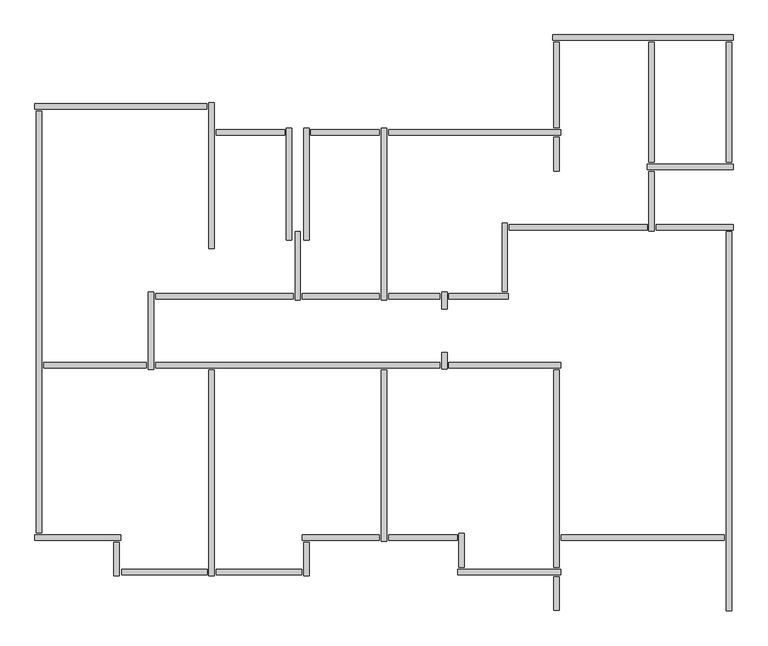
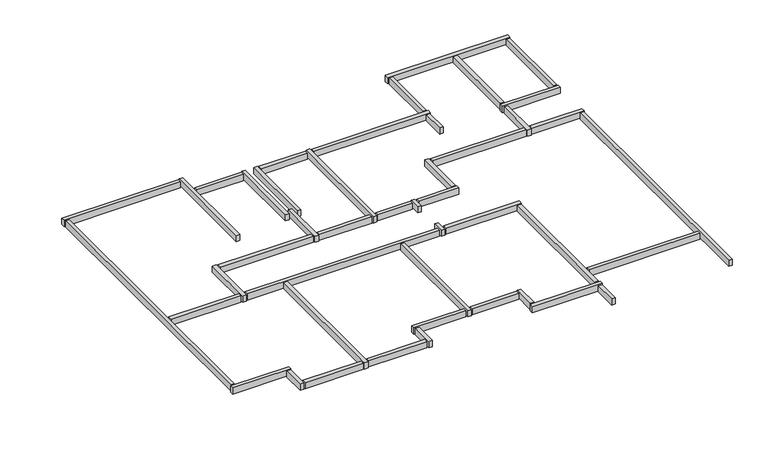
"""IFC4 building model written with IfcOpenShell, lengths in millimetres: beam geometry, Graute viga de respaldo18 : Graute viga de respaldo."""

import ifcopenshell
import ifcopenshell.guid

model = None  # the IFC model being written
_history = None  # IfcOwnerHistory: only IFC2X3 demands one
_inside = {}  # id of a spatial element -> (the spatial element, [elements in it])
_under = {}  # id of a project, library or spatial element -> (it, [spatial elements below it])
_declared = {}  # id of a project -> (the project, [libraries it declares])
_typed = {}  # id of a type object -> (the type object, [elements of that type])
_made_of = {}  # id of a material, layer set ... -> (it, [elements and type objects made of it])


def new_model(schema):
    """Start an empty IFC model of exactly this schema.

    Asked for "IFC4X3", IfcOpenShell would pick the latest addendum, in which some entities
    have other attributes; the version numbers below select the first issue.
    IFC2X3 requires an IfcOwnerHistory on every rooted entity: one is made here for all.
    """
    global model, _history
    if schema == "IFC4X3":
        model = ifcopenshell.file(schema_version=(4, 3, 0, 0))
    else:
        model = ifcopenshell.file(schema=schema)
    _inside.clear()
    _under.clear()
    _declared.clear()
    _typed.clear()
    _made_of.clear()
    _history = None
    if model.schema == "IFC2X3":
        org = make("IfcOrganization", Name="unknown")
        user = make(
            "IfcPersonAndOrganization",
            ThePerson=make("IfcPerson", FamilyName="unknown"),
            TheOrganization=org,
        )
        app = make(
            "IfcApplication",
            ApplicationDeveloper=org,
            Version="unknown",
            ApplicationFullName="unknown",
            ApplicationIdentifier="unknown",
        )
        _history = make(
            "IfcOwnerHistory",
            OwningUser=user,
            OwningApplication=app,
            ChangeAction="ADDED",
            CreationDate=0,
        )
    return model


def make(cls, **values):
    """One entity of the class cls with the attributes given. An attribute that is None is left unset."""
    return model.create_entity(
        cls, **{name: value for name, value in values.items() if value is not None}
    )


def rooted(cls, **values):
    """An entity with a GlobalId (a new one), such as an element, a storey or a relation."""
    return make(cls, GlobalId=ifcopenshell.guid.new(), OwnerHistory=_history, **values)


def si_unit(unit_type, name, prefix=None):
    """IfcSIUnit, for example si_unit("LENGTHUNIT", "METRE", prefix="MILLI")."""
    return make("IfcSIUnit", UnitType=unit_type, Prefix=prefix, Name=name)


def assignment(units):
    """IfcUnitAssignment: the units of a project."""
    return None if units is None else make("IfcUnitAssignment", Units=units)


def point(xyz):
    """IfcCartesianPoint."""
    return None if xyz is None else make("IfcCartesianPoint", Coordinates=xyz)


def direction(xyz):
    """IfcDirection."""
    return None if xyz is None else make("IfcDirection", DirectionRatios=xyz)


def frame(location, z_axis=None, x_axis=None):
    """IfcAxis2Placement3D, a coordinate frame: its origin and axes. An axis left out is left unset."""
    return make(
        "IfcAxis2Placement3D",
        Location=point(location),
        Axis=direction(z_axis),
        RefDirection=direction(x_axis),
    )


def origin():
    """The frame at (0, 0, 0) with its axes left unset."""
    return frame((0.0, 0.0, 0.0))


def place(relative_to, where):
    """IfcLocalPlacement: puts the frame where relative to a parent placement (None: the world)."""
    return make(
        "IfcLocalPlacement", PlacementRelTo=relative_to, RelativePlacement=where
    )


def context(
    kind, dimensions, precision=None, world=None, true_north=None, identifier=None
):
    """IfcGeometricRepresentationContext, for example the 3D "Model" context."""
    return make(
        "IfcGeometricRepresentationContext",
        ContextIdentifier=identifier,
        ContextType=kind,
        CoordinateSpaceDimension=dimensions,
        Precision=precision,
        WorldCoordinateSystem=world,
        TrueNorth=true_north,
    )


def project(units=None, contexts=None):
    """IfcProject with its units and contexts."""
    return rooted(
        "IfcProject",
        Name="project",
        RepresentationContexts=contexts,
        UnitsInContext=assignment(units),
    )


def spatial(cls, under=None, at=None, **own):
    """A site, building, storey or space (cls), placed at a placement, below another one or the project."""
    s = rooted(cls, ObjectPlacement=at, **own)
    if under is not None:
        _under.setdefault(under.id(), (under, []))[1].append(s)
    return s


def polyline(points):
    """IfcPolyline through the points."""
    return make("IfcPolyline", Points=[point(p) for p in points])


def outline(outer, holes=None, kind="AREA"):
    """IfcArbitraryClosedProfileDef: a profile drawn as a closed curve; with holes, ...WithVoids."""
    if holes is None:
        return make("IfcArbitraryClosedProfileDef", ProfileType=kind, OuterCurve=outer)
    return make(
        "IfcArbitraryProfileDefWithVoids",
        ProfileType=kind,
        OuterCurve=outer,
        InnerCurves=holes,
    )


def extrude(swept, where, along, depth):
    """IfcExtrudedAreaSolid: the profile swept, set in the frame where, extruded along a direction by depth."""
    return make(
        "IfcExtrudedAreaSolid",
        SweptArea=swept,
        Position=where,
        ExtrudedDirection=direction(along),
        Depth=depth,
    )


def shape(context_of_items, identifier, shape_type, items):
    """IfcShapeRepresentation: the items that make up one representation, for example the "Body"."""
    return make(
        "IfcShapeRepresentation",
        ContextOfItems=context_of_items,
        RepresentationIdentifier=identifier,
        RepresentationType=shape_type,
        Items=items,
    )


def source(mapping_origin, context_of_items, identifier, shape_type, items):
    """IfcRepresentationMap: a shape defined once, which mapped items show again and again."""
    return make(
        "IfcRepresentationMap",
        MappingOrigin=mapping_origin,
        MappedRepresentation=shape(context_of_items, identifier, shape_type, items),
    )


def transform(
    local_origin,
    x_axis=None,
    y_axis=None,
    z_axis=None,
    scale=None,
    scale2=None,
    scale3=None,
    uniform=True,
):
    """IfcCartesianTransformationOperator3D, or its non-uniform kind. x_axis, y_axis, z_axis: its Axis1, 2, 3."""
    if uniform:
        return make(
            "IfcCartesianTransformationOperator3D",
            Axis1=direction(x_axis),
            Axis2=direction(y_axis),
            LocalOrigin=point(local_origin),
            Scale=scale,
            Axis3=direction(z_axis),
        )
    return make(
        "IfcCartesianTransformationOperator3DnonUniform",
        Axis1=direction(x_axis),
        Axis2=direction(y_axis),
        LocalOrigin=point(local_origin),
        Scale=scale,
        Axis3=direction(z_axis),
        Scale2=scale2,
        Scale3=scale3,
    )


def mapped(mapping_source, mapping_target):
    """IfcMappedItem: shows the shape of a source again, moved by a transform."""
    return make(
        "IfcMappedItem", MappingSource=mapping_source, MappingTarget=mapping_target
    )


def made_of(thing, what):
    """Note that an element or type object is made of a material, layer set ...; save() writes the relation."""
    if what is not None:
        _made_of.setdefault(what.id(), (what, []))[1].append(thing)
    return thing


def element(
    cls,
    number,
    at=None,
    inside=None,
    cuts=None,
    type_object=None,
    material=None,
    context=None,
    identifier="Body",
    shape_type=None,
    held_by="IfcProductDefinitionShape",
    body=None,
    shapes=None,
    **own,
):
    """One element of the class cls, such as IfcWall. Its Tag is "e" and its number.

    at: its placement. inside: the storey or other place that contains it. cuts: it is an
    opening in that element (IfcRelVoidsElement). A single representation is given by context,
    identifier, shape_type and body (its items); several are given by shapes. held_by: the class
    of the entity that holds the representations. save() writes the other relations.
    """
    e = rooted(cls, Tag="e%d" % number, ObjectPlacement=at, **own)
    if body is not None:
        shapes = [shape(context, identifier, shape_type, body)]
    if shapes is not None:
        e.Representation = make(held_by, Representations=shapes)
    if inside is not None:
        _inside.setdefault(inside.id(), (inside, []))[1].append(e)
    if cuts is not None:
        rooted(
            "IfcRelVoidsElement", RelatingBuildingElement=cuts, RelatedOpeningElement=e
        )
    if type_object is not None:
        _typed.setdefault(type_object.id(), (type_object, []))[1].append(e)
    return made_of(e, material)


def aggregate(whole, parts):
    """IfcRelAggregates: a whole, such as a stair, and the parts it consists of."""
    return rooted("IfcRelAggregates", RelatingObject=whole, RelatedObjects=parts)


def save(model, path):
    """Write the relations noted so far, then the file.

    IfcRelAggregates (storeys below a building ...), IfcRelContainedInSpatialStructure (elements
    in a storey), IfcRelDefinesByType, IfcRelAssociatesMaterial and IfcRelDeclares: one each for
    every whole, place, type object, material and project.
    """
    for whole, parts in _under.values():
        aggregate(whole, parts)
    for where, things in _inside.values():
        rooted(
            "IfcRelContainedInSpatialStructure",
            RelatedElements=things,
            RelatingStructure=where,
        )
    for kind, things in _typed.values():
        rooted("IfcRelDefinesByType", RelatedObjects=things, RelatingType=kind)
    for what, things in _made_of.values():
        rooted("IfcRelAssociatesMaterial", RelatedObjects=things, RelatingMaterial=what)
    for by, libraries in _declared.values():
        rooted("IfcRelDeclares", RelatingContext=by, RelatedDefinitions=libraries)
    model.write(path)


def beam_be0dcb32(model_context):
    return source(origin(), model_context, "Body", "SweptSolid", [
        extrude(outline(polyline([(-75401.7587292, 57502.4278788), (-75401.7587292, 57408.4278788), (-76591.7587292, 57408.4278788), (-76591.7587292, 57502.4278788), (-75401.7587292, 57502.4278788)])), frame((0.0, 0.0, 14632.9999999), z_axis=(0.0, 0.0, 1.0), x_axis=(1.0, 0.0, 0.0)), (0.0, 0.0, 1.0), 167.0),
        extrude(outline(polyline([(-73751.7587292, 57502.4278788), (-73751.7587292, 57408.4278788), (-74941.7587292, 57408.4278788), (-74941.7587292, 57502.4278788), (-73751.7587292, 57502.4278788)])), frame((0.0, 0.0, 14632.9999999), z_axis=(0.0, 0.0, 1.0), x_axis=(1.0, 0.0, 0.0)), (0.0, 0.0, 1.0), 167.0),
        extrude(outline(polyline([(-77801.7587292, 53452.4278788), (-77801.7587292, 53358.4278788), (-79591.7587292, 53358.4278788), (-79591.7587292, 53452.4278788), (-77801.7587292, 53452.4278788)])), frame((0.0, 0.0, 14632.9999999), z_axis=(0.0, 0.0, 1.0), x_axis=(1.0, 0.0, 0.0)), (0.0, 0.0, 1.0), 167.0),
        extrude(outline(polyline([(-72401.7587292, 50452.4278788), (-72401.7587292, 50358.4278788), (-73591.7587292, 50358.4278788), (-73591.7587292, 50452.4278788), (-72401.7587292, 50452.4278788)])), frame((0.0, 0.0, 14632.9999999), z_axis=(0.0, 0.0, 1.0), x_axis=(1.0, 0.0, 0.0)), (0.0, 0.0, 1.0), 167.0),
        extrude(outline(polyline([(-72368.7587292, 50475.4278788), (-72274.7587292, 50475.4278788), (-72274.7587292, 49885.4278788), (-72368.7587292, 49885.4278788), (-72368.7587292, 50475.4278788)])), frame((0.0, 0.0, 14632.9999999), z_axis=(0.0, 0.0, 1.0), x_axis=(1.0, 0.0, 0.0)), (0.0, 0.0, 1.0), 167.0),
        extrude(outline(polyline([(-70601.7587292, 49852.4278788), (-70601.7587292, 49758.4278788), (-72391.7587292, 49758.4278788), (-72391.7587292, 49852.4278788), (-70601.7587292, 49852.4278788)])), frame((0.0, 0.0, 14632.9999999), z_axis=(0.0, 0.0, 1.0), x_axis=(1.0, 0.0, 0.0)), (0.0, 0.0, 1.0), 167.0),
        extrude(outline(polyline([(-72574.7587292, 53335.4278788), (-72668.7587292, 53335.4278788), (-72668.7587292, 53625.4278788), (-72574.7587292, 53625.4278788), (-72574.7587292, 53335.4278788)])), frame((0.0, 0.0, 14632.9999999), z_axis=(0.0, 0.0, 1.0), x_axis=(1.0, 0.0, 0.0)), (0.0, 0.0, 1.0), 167.0),
        extrude(outline(polyline([(-75251.7587292, 54652.4278788), (-75251.7587292, 54558.4278788), (-77641.7587292, 54558.4278788), (-77641.7587292, 54652.4278788), (-75251.7587292, 54652.4278788)])), frame((0.0, 0.0, 14632.9999999), z_axis=(0.0, 0.0, 1.0), x_axis=(1.0, 0.0, 0.0)), (0.0, 0.0, 1.0), 167.0),
        extrude(outline(polyline([(-73751.7587292, 54652.4278788), (-73751.7587292, 54558.4278788), (-75091.7587292, 54558.4278788), (-75091.7587292, 54652.4278788), (-73751.7587292, 54652.4278788)])), frame((0.0, 0.0, 14632.9999999), z_axis=(0.0, 0.0, 1.0), x_axis=(1.0, 0.0, 0.0)), (0.0, 0.0, 1.0), 167.0),
        extrude(outline(polyline([(-72701.7587292, 54652.4278788), (-72701.7587292, 54558.4278788), (-73591.7587292, 54558.4278788), (-73591.7587292, 54652.4278788), (-72701.7587292, 54652.4278788)])), frame((0.0, 0.0, 14632.9999999), z_axis=(0.0, 0.0, 1.0), x_axis=(1.0, 0.0, 0.0)), (0.0, 0.0, 1.0), 167.0),
        extrude(outline(polyline([(-72574.7587292, 54385.4278788), (-72668.7587292, 54385.4278788), (-72668.7587292, 54675.4278788), (-72574.7587292, 54675.4278788), (-72574.7587292, 54385.4278788)])), frame((0.0, 0.0, 14632.9999999), z_axis=(0.0, 0.0, 1.0), x_axis=(1.0, 0.0, 0.0)), (0.0, 0.0, 1.0), 167.0),
        extrude(outline(polyline([(-71511.7587292, 54652.4278788), (-71511.7587292, 54558.4278788), (-72541.7587292, 54558.4278788), (-72541.7587292, 54652.4278788), (-71511.7587292, 54652.4278788)])), frame((0.0, 0.0, 14632.9999999), z_axis=(0.0, 0.0, 1.0), x_axis=(1.0, 0.0, 0.0)), (0.0, 0.0, 1.0), 167.0),
        extrude(outline(polyline([(-71618.7587292, 55875.4278788), (-71524.7587292, 55875.4278788), (-71524.7587292, 54685.4278788), (-71618.7587292, 54685.4278788), (-71618.7587292, 55875.4278788)])), frame((0.0, 0.0, 14632.9999999), z_axis=(0.0, 0.0, 1.0), x_axis=(1.0, 0.0, 0.0)), (0.0, 0.0, 1.0), 167.0),
        extrude(outline(polyline([(-69091.7587292, 55852.4278788), (-69091.7587292, 55758.4278788), (-71491.7587292, 55758.4278788), (-71491.7587292, 55852.4278788), (-69091.7587292, 55852.4278788)])), frame((0.0, 0.0, 14632.9999999), z_axis=(0.0, 0.0, 1.0), x_axis=(1.0, 0.0, 0.0)), (0.0, 0.0, 1.0), 167.0),
        extrude(outline(polyline([(-73624.7587292, 54540.4278788), (-73718.7587292, 54540.4278788), (-73718.7587292, 57525.4278788), (-73624.7587292, 57525.4278788), (-73624.7587292, 54540.4278788)])), frame((0.0, 0.0, 14632.9999999), z_axis=(0.0, 0.0, 1.0), x_axis=(1.0, 0.0, 0.0)), (0.0, 0.0, 1.0), 167.0),
        extrude(outline(polyline([(-70601.7587292, 57502.4278788), (-70601.7587292, 57408.4278788), (-73591.7587292, 57408.4278788), (-73591.7587292, 57502.4278788), (-70601.7587292, 57502.4278788)])), frame((0.0, 0.0, 14632.9999999), z_axis=(0.0, 0.0, 1.0), x_axis=(1.0, 0.0, 0.0)), (0.0, 0.0, 1.0), 167.0),
        extrude(outline(polyline([(-70624.7587292, 56785.4278788), (-70718.7587292, 56785.4278788), (-70718.7587292, 57375.4278788), (-70624.7587292, 57375.4278788), (-70624.7587292, 56785.4278788)])), frame((0.0, 0.0, 14632.9999999), z_axis=(0.0, 0.0, 1.0), x_axis=(1.0, 0.0, 0.0)), (0.0, 0.0, 1.0), 167.0),
        extrude(outline(polyline([(-70718.7587292, 59025.4278788), (-70624.7587292, 59025.4278788), (-70624.7587292, 57535.4278788), (-70718.7587292, 57535.4278788), (-70718.7587292, 59025.4278788)])), frame((0.0, 0.0, 14632.9999999), z_axis=(0.0, 0.0, 1.0), x_axis=(1.0, 0.0, 0.0)), (0.0, 0.0, 1.0), 167.0),
        extrude(outline(polyline([(-67718.7587292, 59025.4278788), (-67624.7587292, 59025.4278788), (-67624.7587292, 56935.4278788), (-67718.7587292, 56935.4278788), (-67718.7587292, 59025.4278788)])), frame((0.0, 0.0, 14632.9999999), z_axis=(0.0, 0.0, 1.0), x_axis=(1.0, 0.0, 0.0)), (0.0, 0.0, 1.0), 167.0),
        extrude(outline(polyline([(-69068.7587292, 59025.4278788), (-68974.7587292, 59025.4278788), (-68974.7587292, 56935.4278788), (-69068.7587292, 56935.4278788), (-69068.7587292, 59025.4278788)])), frame((0.0, 0.0, 14632.9999999), z_axis=(0.0, 0.0, 1.0), x_axis=(1.0, 0.0, 0.0)), (0.0, 0.0, 1.0), 167.0),
        extrude(outline(polyline([(-68974.7587292, 55735.4278788), (-69068.7587292, 55735.4278788), (-69068.7587292, 56775.4278788), (-68974.7587292, 56775.4278788), (-68974.7587292, 55735.4278788)])), frame((0.0, 0.0, 14632.9999999), z_axis=(0.0, 0.0, 1.0), x_axis=(1.0, 0.0, 0.0)), (0.0, 0.0, 1.0), 167.0),
        extrude(outline(polyline([(-67751.7587292, 50452.4278788), (-67751.7587292, 50358.4278788), (-70591.7587292, 50358.4278788), (-70591.7587292, 50452.4278788), (-67751.7587292, 50452.4278788)])), frame((0.0, 0.0, 14632.9999999), z_axis=(0.0, 0.0, 1.0), x_axis=(1.0, 0.0, 0.0)), (0.0, 0.0, 1.0), 167.0),
        extrude(outline(polyline([(-70718.7587292, 53325.4278788), (-70624.7587292, 53325.4278788), (-70624.7587292, 49885.4278788), (-70718.7587292, 49885.4278788), (-70718.7587292, 53325.4278788)])), frame((0.0, 0.0, 14632.9999999), z_axis=(0.0, 0.0, 1.0), x_axis=(1.0, 0.0, 0.0)), (0.0, 0.0, 1.0), 167.0),
        extrude(outline(polyline([(-70601.7587292, 53452.4278788), (-70601.7587292, 53358.4278788), (-72541.7587292, 53358.4278788), (-72541.7587292, 53452.4278788), (-70601.7587292, 53452.4278788)])), frame((0.0, 0.0, 14632.9999999), z_axis=(0.0, 0.0, 1.0), x_axis=(1.0, 0.0, 0.0)), (0.0, 0.0, 1.0), 167.0),
        extrude(outline(polyline([(-72701.7587292, 53452.4278788), (-72701.7587292, 53358.4278788), (-77641.7587292, 53358.4278788), (-77641.7587292, 53452.4278788), (-72701.7587292, 53452.4278788)])), frame((0.0, 0.0, 14632.9999999), z_axis=(0.0, 0.0, 1.0), x_axis=(1.0, 0.0, 0.0)), (0.0, 0.0, 1.0), 167.0),
        extrude(outline(polyline([(-73624.7587292, 50335.4278788), (-73718.7587292, 50335.4278788), (-73718.7587292, 53325.4278788), (-73624.7587292, 53325.4278788), (-73624.7587292, 50335.4278788)])), frame((0.0, 0.0, 14632.9999999), z_axis=(0.0, 0.0, 1.0), x_axis=(1.0, 0.0, 0.0)), (0.0, 0.0, 1.0), 167.0),
        extrude(outline(polyline([(-75091.7587292, 50358.4278788), (-75091.7587292, 50452.4278788), (-73751.7587292, 50452.4278788), (-73751.7587292, 50358.4278788), (-75091.7587292, 50358.4278788)])), frame((0.0, 0.0, 14632.9999999), z_axis=(0.0, 0.0, 1.0), x_axis=(1.0, 0.0, 0.0)), (0.0, 0.0, 1.0), 167.0),
        extrude(outline(polyline([(-74974.7587292, 49735.4278788), (-75068.7587292, 49735.4278788), (-75068.7587292, 50325.4278788), (-74974.7587292, 50325.4278788), (-74974.7587292, 49735.4278788)])), frame((0.0, 0.0, 14632.9999999), z_axis=(0.0, 0.0, 1.0), x_axis=(1.0, 0.0, 0.0)), (0.0, 0.0, 1.0), 167.0),
        extrude(outline(polyline([(-75101.7587292, 49852.4278788), (-75101.7587292, 49758.4278788), (-76591.7587292, 49758.4278788), (-76591.7587292, 49852.4278788), (-75101.7587292, 49852.4278788)])), frame((0.0, 0.0, 14632.9999999), z_axis=(0.0, 0.0, 1.0), x_axis=(1.0, 0.0, 0.0)), (0.0, 0.0, 1.0), 167.0),
        extrude(outline(polyline([(-78230.736554, 49758.4278788), (-78230.736554, 49853.4278788), (-76741.7587292, 49853.4278788), (-76741.7587292, 49758.4278788), (-78230.736554, 49758.4278788)])), frame((0.0, 0.0, 14617.1856208), z_axis=(0.0, 0.0, 1.0), x_axis=(1.0, 0.0, 0.0)), (0.0, 0.0, 1.0), 165.0),
        extrude(outline(polyline([(-79718.7587292, 57825.4278788), (-79624.7587292, 57825.4278788), (-79624.7587292, 50485.4278788), (-79718.7587292, 50485.4278788), (-79718.7587292, 57825.4278788)])), frame((0.0, 0.0, 14632.9999999), z_axis=(0.0, 0.0, 1.0), x_axis=(1.0, 0.0, 0.0)), (0.0, 0.0, 1.0), 167.0),
        extrude(outline(polyline([(-77768.7587292, 54675.4278788), (-77674.7587292, 54675.4278788), (-77674.7587292, 53330.0746661), (-77768.7587292, 53330.0746661), (-77768.7587292, 54675.4278788)])), frame((0.0, 0.0, 14632.9999999), z_axis=(0.0, 0.0, 1.0), x_axis=(1.0, 0.0, 0.0)), (0.0, 0.0, 1.0), 167.0),
        extrude(outline(polyline([(-75218.7587292, 55725.4278788), (-75124.7587292, 55725.4278788), (-75124.7587292, 54535.4278788), (-75218.7587292, 54535.4278788), (-75218.7587292, 55725.4278788)])), frame((0.0, 0.0, 14632.9999999), z_axis=(0.0, 0.0, 1.0), x_axis=(1.0, 0.0, 0.0)), (0.0, 0.0, 1.0), 167.0),
        extrude(outline(polyline([(-75368.7587292, 57525.4278788), (-75274.7587292, 57525.4278788), (-75274.7587292, 55585.4278788), (-75368.7587292, 55585.4278788), (-75368.7587292, 57525.4278788)])), frame((0.0, 0.0, 14632.9999999), z_axis=(0.0, 0.0, 1.0), x_axis=(1.0, 0.0, 0.0)), (0.0, 0.0, 1.0), 167.0),
        extrude(outline(polyline([(-75068.7587292, 57525.4278788), (-74974.7587292, 57525.4278788), (-74974.7587292, 55585.4278788), (-75068.7587292, 55585.4278788), (-75068.7587292, 57525.4278788)])), frame((0.0, 0.0, 14632.9999999), z_axis=(0.0, 0.0, 1.0), x_axis=(1.0, 0.0, 0.0)), (0.0, 0.0, 1.0), 167.0),
        extrude(outline(polyline([(-76718.7587292, 57975.4278788), (-76624.7587292, 57975.4278788), (-76624.7587292, 55435.4278788), (-76718.7587292, 55435.4278788), (-76718.7587292, 57975.4278788)])), frame((0.0, 0.0, 14632.9999999), z_axis=(0.0, 0.0, 1.0), x_axis=(1.0, 0.0, 0.0)), (0.0, 0.0, 1.0), 167.0),
        extrude(outline(polyline([(-79741.7587292, 57858.4278788), (-79741.7587292, 57952.4278788), (-76751.7587292, 57952.4278788), (-76751.7587292, 57858.4278788), (-79741.7587292, 57858.4278788)])), frame((0.0, 0.0, 14632.9999999), z_axis=(0.0, 0.0, 1.0), x_axis=(1.0, 0.0, 0.0)), (0.0, 0.0, 1.0), 167.0),
        extrude(outline(polyline([(-78274.7587292, 49735.4278788), (-78368.7587292, 49735.4278788), (-78368.7587292, 50325.4278788), (-78274.7587292, 50325.4278788), (-78274.7587292, 49735.4278788)])), frame((0.0, 0.0, 14632.9999999), z_axis=(0.0, 0.0, 1.0), x_axis=(1.0, 0.0, 0.0)), (0.0, 0.0, 1.0), 167.0),
        extrude(outline(polyline([(-78251.7587292, 50452.4278788), (-78251.7587292, 50358.4278788), (-79741.7587292, 50358.4278788), (-79741.7587292, 50452.4278788), (-78251.7587292, 50452.4278788)])), frame((0.0, 0.0, 14632.9999999), z_axis=(0.0, 0.0, 1.0), x_axis=(1.0, 0.0, 0.0)), (0.0, 0.0, 1.0), 167.0),
        extrude(outline(polyline([(-76624.7587292, 49735.4278788), (-76718.7587292, 49735.4278788), (-76718.7587292, 53325.4278788), (-76624.7587292, 53325.4278788), (-76624.7587292, 49735.4278788)])), frame((0.0, 0.0, 14632.9999999), z_axis=(0.0, 0.0, 1.0), x_axis=(1.0, 0.0, 0.0)), (0.0, 0.0, 1.0), 167.0),
        extrude(outline(polyline([(-70624.7587292, 49135.4278788), (-70718.7587292, 49135.4278788), (-70718.7587292, 49725.4278788), (-70624.7587292, 49725.4278788), (-70624.7587292, 49135.4278788)])), frame((0.0, 0.0, 14632.9999999), z_axis=(0.0, 0.0, 1.0), x_axis=(1.0, 0.0, 0.0)), (0.0, 0.0, 1.0), 167.0),
        extrude(outline(polyline([(-67601.7587292, 56902.4278788), (-67601.7587292, 56808.4278788), (-69091.7587292, 56808.4278788), (-69091.7587292, 56902.4278788), (-67601.7587292, 56902.4278788)])), frame((0.0, 0.0, 14632.9999999), z_axis=(0.0, 0.0, 1.0), x_axis=(1.0, 0.0, 0.0)), (0.0, 0.0, 1.0), 167.0),
        extrude(outline(polyline([(-67601.7587292, 59152.4278788), (-67601.7587292, 59058.4278788), (-70741.7587292, 59058.4278788), (-70741.7587292, 59152.4278788), (-67601.7587292, 59152.4278788)])), frame((0.0, 0.0, 14632.9999999), z_axis=(0.0, 0.0, 1.0), x_axis=(1.0, 0.0, 0.0)), (0.0, 0.0, 1.0), 167.0),
        extrude(outline(polyline([(-67601.7587292, 55852.4278788), (-67601.7587292, 55758.4278788), (-68941.7587292, 55758.4278788), (-68941.7587292, 55852.4278788), (-67601.7587292, 55852.4278788)])), frame((0.0, 0.0, 14632.9999999), z_axis=(0.0, 0.0, 1.0), x_axis=(1.0, 0.0, 0.0)), (0.0, 0.0, 1.0), 167.0),
        extrude(outline(polyline([(-67624.7587292, 49132.8979841), (-67718.7587292, 49132.8979841), (-67718.7587292, 55725.4278788), (-67624.7587292, 55725.4278788), (-67624.7587292, 49132.8979841)])), frame((0.0, 0.0, 14632.9999999), z_axis=(0.0, 0.0, 1.0), x_axis=(1.0, 0.0, 0.0)), (0.0, 0.0, 1.0), 167.0),
    ])


if __name__ == "__main__":
    model = new_model("IFC4")
    model_context = context("Model", 3, world=origin())
    ifc_project = project(units=[si_unit("LENGTHUNIT", "METRE", prefix="MILLI")], contexts=[model_context])
    site = spatial("IfcSite", under=ifc_project)
    building = spatial("IfcBuilding", under=site)
    placement = place(None, origin())
    beam_shape = beam_be0dcb32(model_context)
    element("IfcBeam", 1, ObjectType="Graute viga de respaldo18 : Graute viga de respaldo", at=placement, inside=building, context=model_context, shape_type="MappedRepresentation", body=[
        mapped(beam_shape, transform((0.0, 0.0, 0.0), x_axis=(1.0, 0.0, 0.0), y_axis=(0.0, 1.0, 0.0), z_axis=(0.0, 0.0, 1.0))),
    ])
    save(model, "model.ifc")

# Revit data of these elements
# Element 1 (IfcBeam, "Graute viga de respaldo18 : Graute viga de respaldo")
#   Materials on its faces: "Concreto, Faixa de areia/cimento"
# Materials
#   "Concreto, Faixa de areia/cimento": class "Concreto", colour RGB 127 127 127, transparency 0, Description = "Revestimento de laje de concreto", Cost = 0
